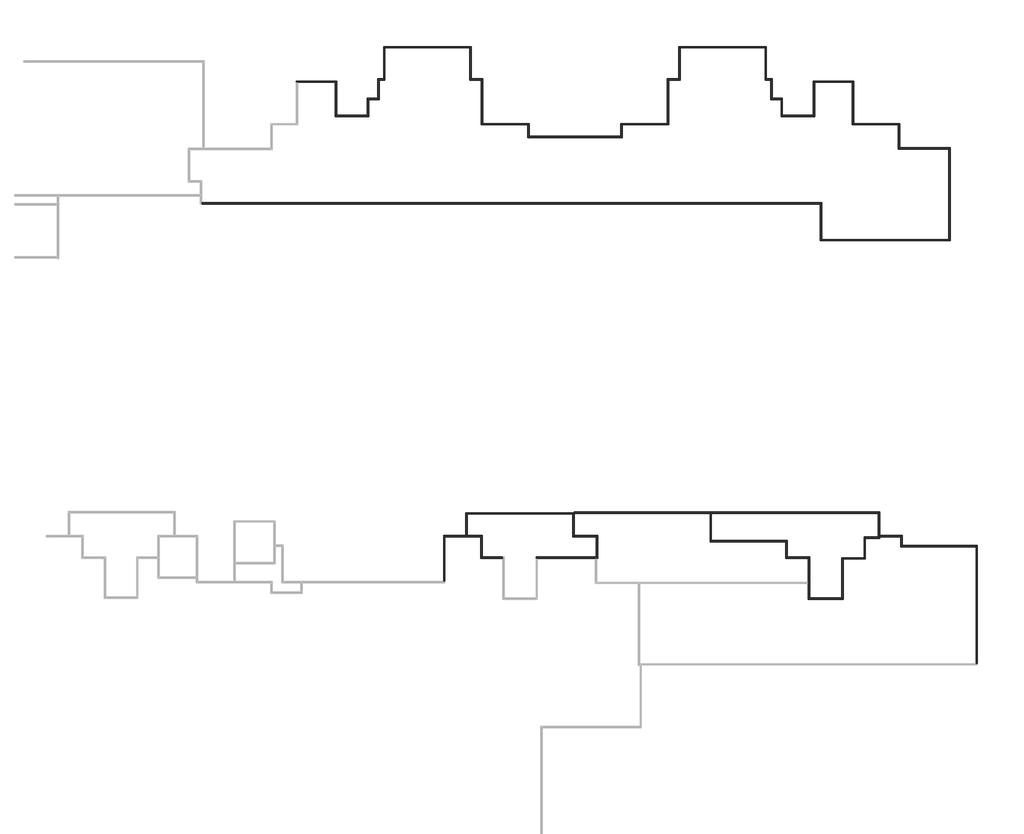
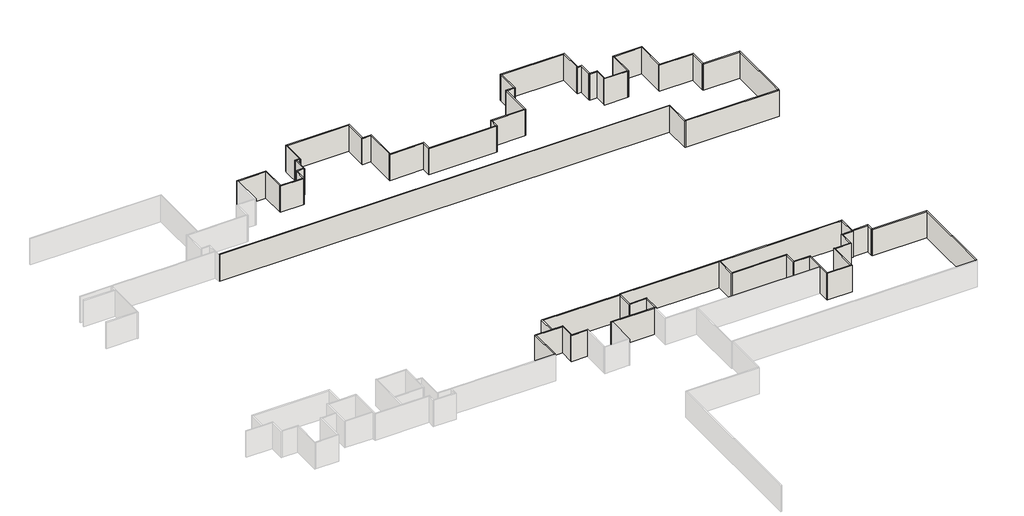
# One storey, part 8 of 8: 63 walls.
"""IFC4 building model written with IfcOpenShell, lengths in millimetres."""

import ifcopenshell
import ifcopenshell.guid

model = None  # the IFC model being written
_history = None  # IfcOwnerHistory: only IFC2X3 demands one
_inside = {}  # id of a spatial element -> (the spatial element, [elements in it])
_under = {}  # id of a project, library or spatial element -> (it, [spatial elements below it])
_declared = {}  # id of a project -> (the project, [libraries it declares])
_typed = {}  # id of a type object -> (the type object, [elements of that type])
_made_of = {}  # id of a material, layer set ... -> (it, [elements and type objects made of it])


def new_model(schema):
    """Start an empty IFC model of exactly this schema.

    Asked for "IFC4X3", IfcOpenShell would pick the latest addendum, in which some entities
    have other attributes; the version numbers below select the first issue.
    IFC2X3 requires an IfcOwnerHistory on every rooted entity: one is made here for all.
    """
    global model, _history
    if schema == "IFC4X3":
        model = ifcopenshell.file(schema_version=(4, 3, 0, 0))
    else:
        model = ifcopenshell.file(schema=schema)
    _inside.clear()
    _under.clear()
    _declared.clear()
    _typed.clear()
    _made_of.clear()
    _history = None
    if model.schema == "IFC2X3":
        org = make("IfcOrganization", Name="unknown")
        user = make(
            "IfcPersonAndOrganization",
            ThePerson=make("IfcPerson", FamilyName="unknown"),
            TheOrganization=org,
        )
        app = make(
            "IfcApplication",
            ApplicationDeveloper=org,
            Version="unknown",
            ApplicationFullName="unknown",
            ApplicationIdentifier="unknown",
        )
        _history = make(
            "IfcOwnerHistory",
            OwningUser=user,
            OwningApplication=app,
            ChangeAction="ADDED",
            CreationDate=0,
        )
    return model


def make(cls, **values):
    """One entity of the class cls with the attributes given. An attribute that is None is left unset."""
    return model.create_entity(
        cls, **{name: value for name, value in values.items() if value is not None}
    )


def rooted(cls, **values):
    """An entity with a GlobalId (a new one), such as an element, a storey or a relation."""
    return make(cls, GlobalId=ifcopenshell.guid.new(), OwnerHistory=_history, **values)


def si_unit(unit_type, name, prefix=None):
    """IfcSIUnit, for example si_unit("LENGTHUNIT", "METRE", prefix="MILLI")."""
    return make("IfcSIUnit", UnitType=unit_type, Prefix=prefix, Name=name)


def assignment(units):
    """IfcUnitAssignment: the units of a project."""
    return None if units is None else make("IfcUnitAssignment", Units=units)


def point(xyz):
    """IfcCartesianPoint."""
    return None if xyz is None else make("IfcCartesianPoint", Coordinates=xyz)


def direction(xyz):
    """IfcDirection."""
    return None if xyz is None else make("IfcDirection", DirectionRatios=xyz)


def frame(location, z_axis=None, x_axis=None):
    """IfcAxis2Placement3D, a coordinate frame: its origin and axes. An axis left out is left unset."""
    return make(
        "IfcAxis2Placement3D",
        Location=point(location),
        Axis=direction(z_axis),
        RefDirection=direction(x_axis),
    )


def origin():
    """The frame at (0, 0, 0) with its axes left unset."""
    return frame((0.0, 0.0, 0.0))


def origin_with_axes():
    """The frame at (0, 0, 0) with the z axis (0, 0, 1) and the x axis (1, 0, 0) written out."""
    return frame((0.0, 0.0, 0.0), z_axis=(0.0, 0.0, 1.0), x_axis=(1.0, 0.0, 0.0))


def place(relative_to, where):
    """IfcLocalPlacement: puts the frame where relative to a parent placement (None: the world)."""
    return make(
        "IfcLocalPlacement", PlacementRelTo=relative_to, RelativePlacement=where
    )


def context(
    kind, dimensions, precision=None, world=None, true_north=None, identifier=None
):
    """IfcGeometricRepresentationContext, for example the 3D "Model" context."""
    return make(
        "IfcGeometricRepresentationContext",
        ContextIdentifier=identifier,
        ContextType=kind,
        CoordinateSpaceDimension=dimensions,
        Precision=precision,
        WorldCoordinateSystem=world,
        TrueNorth=true_north,
    )


def project(units=None, contexts=None):
    """IfcProject with its units and contexts."""
    return rooted(
        "IfcProject",
        Name="project",
        RepresentationContexts=contexts,
        UnitsInContext=assignment(units),
    )


def spatial(cls, under=None, at=None, **own):
    """A site, building, storey or space (cls), placed at a placement, below another one or the project."""
    s = rooted(cls, ObjectPlacement=at, **own)
    if under is not None:
        _under.setdefault(under.id(), (under, []))[1].append(s)
    return s


def polyline(points):
    """IfcPolyline through the points."""
    return make("IfcPolyline", Points=[point(p) for p in points])


def outline(outer, holes=None, kind="AREA"):
    """IfcArbitraryClosedProfileDef: a profile drawn as a closed curve; with holes, ...WithVoids."""
    if holes is None:
        return make("IfcArbitraryClosedProfileDef", ProfileType=kind, OuterCurve=outer)
    return make(
        "IfcArbitraryProfileDefWithVoids",
        ProfileType=kind,
        OuterCurve=outer,
        InnerCurves=holes,
    )


def extrude(swept, where, along, depth):
    """IfcExtrudedAreaSolid: the profile swept, set in the frame where, extruded along a direction by depth."""
    return make(
        "IfcExtrudedAreaSolid",
        SweptArea=swept,
        Position=where,
        ExtrudedDirection=direction(along),
        Depth=depth,
    )


def faces_of(points, faces, orient=None, outer=None):
    """IfcFace entities. A face is a list of loops; a loop is a list of indices into points, from 0.

    orient and outer hold one flag for each loop. By default every Orientation is true, the
    first loop of a face is its IfcFaceOuterBound and the others are IfcFaceBound.
    """
    made = []
    for i, loops in enumerate(faces):
        bounds = []
        for j, loop in enumerate(loops):
            is_outer = j == 0 if outer is None else outer[i][j]
            bounds.append(
                make(
                    "IfcFaceOuterBound" if is_outer else "IfcFaceBound",
                    Bound=make("IfcPolyLoop", Polygon=[points[k] for k in loop]),
                    Orientation=True if orient is None else orient[i][j],
                )
            )
        made.append(make("IfcFace", Bounds=bounds))
    return made


def faceted_brep(points, faces, orient=None, outer=None, voids=None):
    """IfcFacetedBrep: a solid bounded by flat faces; with voids (closed shells), ...WithVoids."""
    shared = [point(p) for p in points]
    hull = make("IfcClosedShell", CfsFaces=faces_of(shared, faces, orient, outer))
    if voids is None:
        return make("IfcFacetedBrep", Outer=hull)
    return make(
        "IfcFacetedBrepWithVoids",
        Outer=hull,
        Voids=[
            make(cls, CfsFaces=faces_of(shared, fs, o, b)) for cls, fs, o, b in voids
        ],
    )


def shape(context_of_items, identifier, shape_type, items):
    """IfcShapeRepresentation: the items that make up one representation, for example the "Body"."""
    return make(
        "IfcShapeRepresentation",
        ContextOfItems=context_of_items,
        RepresentationIdentifier=identifier,
        RepresentationType=shape_type,
        Items=items,
    )


def made_of(thing, what):
    """Note that an element or type object is made of a material, layer set ...; save() writes the relation."""
    if what is not None:
        _made_of.setdefault(what.id(), (what, []))[1].append(thing)
    return thing


def element(
    cls,
    number,
    at=None,
    inside=None,
    cuts=None,
    type_object=None,
    material=None,
    context=None,
    identifier="Body",
    shape_type=None,
    held_by="IfcProductDefinitionShape",
    body=None,
    shapes=None,
    **own,
):
    """One element of the class cls, such as IfcWall. Its Tag is "e" and its number.

    at: its placement. inside: the storey or other place that contains it. cuts: it is an
    opening in that element (IfcRelVoidsElement). A single representation is given by context,
    identifier, shape_type and body (its items); several are given by shapes. held_by: the class
    of the entity that holds the representations. save() writes the other relations.
    """
    e = rooted(cls, Tag="e%d" % number, ObjectPlacement=at, **own)
    if body is not None:
        shapes = [shape(context, identifier, shape_type, body)]
    if shapes is not None:
        e.Representation = make(held_by, Representations=shapes)
    if inside is not None:
        _inside.setdefault(inside.id(), (inside, []))[1].append(e)
    if cuts is not None:
        rooted(
            "IfcRelVoidsElement", RelatingBuildingElement=cuts, RelatedOpeningElement=e
        )
    if type_object is not None:
        _typed.setdefault(type_object.id(), (type_object, []))[1].append(e)
    return made_of(e, material)


def aggregate(whole, parts):
    """IfcRelAggregates: a whole, such as a stair, and the parts it consists of."""
    return rooted("IfcRelAggregates", RelatingObject=whole, RelatedObjects=parts)


def save(model, path):
    """Write the relations noted so far, then the file.

    IfcRelAggregates (storeys below a building ...), IfcRelContainedInSpatialStructure (elements
    in a storey), IfcRelDefinesByType, IfcRelAssociatesMaterial and IfcRelDeclares: one each for
    every whole, place, type object, material and project.
    """
    for whole, parts in _under.values():
        aggregate(whole, parts)
    for where, things in _inside.values():
        rooted(
            "IfcRelContainedInSpatialStructure",
            RelatedElements=things,
            RelatingStructure=where,
        )
    for kind, things in _typed.values():
        rooted("IfcRelDefinesByType", RelatedObjects=things, RelatingType=kind)
    for what, things in _made_of.values():
        rooted("IfcRelAssociatesMaterial", RelatedObjects=things, RelatingMaterial=what)
    for by, libraries in _declared.values():
        rooted("IfcRelDeclares", RelatingContext=by, RelatedDefinitions=libraries)
    model.write(path)


model = new_model("IFC4")

# Units and contexts
model_context = context("Model", 3, world=origin())
ifc_project = project(units=[si_unit("LENGTHUNIT", "METRE", prefix="MILLI")], contexts=[model_context])

# Site, building, storey
site = spatial("IfcSite", under=ifc_project)
building = spatial("IfcBuilding", under=site)
storey = spatial("IfcBuildingStorey", under=building, Name="户型图", Elevation=0.0)

# Walls
placement = place(None, origin())
element("IfcWall", 1, ObjectType="所有墙体", at=placement, inside=storey, context=model_context, shape_type="Brep", body=[
    faceted_brep([(247659.8041272, 127629.6486698, 0.0), (301497.9590704, 127629.6486698, 0.0), (301617.9590704, 127629.6486698, 0.0), (301617.9590704, 127629.6486698, 3300.0), (301497.9590704, 127629.6486698, 3300.0), (247659.8041272, 127629.6486698, 3300.0), (247659.8041272, 127749.6486698, 0.0), (247659.8041272, 127749.6486698, 3300.0), (301617.9590704, 127749.6486698, 3300.0), (301617.9590704, 127749.6486698, 0.0)], [[[0, 1, 2, 3, 4, 5]], [[6, 7, 8, 9]], [[2, 1, 0, 6, 9]], [[5, 4, 3, 8, 7]], [[0, 5, 7, 6]], [[3, 2, 9, 8]]]),
])
element("IfcWall", 2, ObjectType="所有墙体", at=placement, inside=storey, context=model_context, shape_type="Brep", body=[
    faceted_brep([(301497.9590704, 127629.6486698, 0.0), (301497.9590704, 124429.6486698, 0.0), (301497.9590704, 124429.6486698, 3300.0), (301497.9590704, 127629.6486698, 3300.0), (301617.9590704, 127629.6486698, 0.0), (301617.9590704, 127629.6486698, 3300.0), (301617.9590704, 124549.6486698, 3300.0), (301617.9590704, 124429.6486698, 3300.0), (301617.9590704, 124429.6486698, 0.0), (301617.9590704, 124549.6486698, 0.0)], [[[0, 1, 2, 3]], [[4, 5, 6, 7, 8, 9]], [[1, 0, 4, 9, 8]], [[3, 2, 7, 6, 5]], [[0, 3, 5, 4]], [[2, 1, 8, 7]]]),
])
element("IfcWall", 3, ObjectType="所有墙体", at=placement, inside=storey, context=model_context, shape_type="Brep", body=[
    faceted_brep([(301617.9590704, 124429.6486698, 0.0), (312809.8041272, 124429.6486698, 0.0), (312809.8041272, 124429.6486698, 3300.0), (301617.9590704, 124429.6486698, 3300.0), (301617.9590704, 124549.6486698, 0.0), (301617.9590704, 124549.6486698, 3300.0), (312689.8041272, 124549.6486698, 3300.0), (312809.8041272, 124549.6486698, 3300.0), (312809.8041272, 124549.6486698, 0.0), (312689.8041272, 124549.6486698, 0.0)], [[[0, 1, 2, 3]], [[4, 5, 6, 7, 8, 9]], [[1, 0, 4, 9, 8]], [[3, 2, 7, 6, 5]], [[0, 3, 5, 4]], [[2, 1, 8, 7]]]),
])
element("IfcWall", 4, ObjectType="所有墙体", at=placement, inside=storey, context=model_context, shape_type="Brep", body=[
    faceted_brep([(312809.8041272, 124549.6486698, 0.0), (312809.8041272, 132549.6486698, 0.0), (312809.8041272, 132549.6486698, 3300.0), (312809.8041272, 124549.6486698, 3300.0), (312689.8041272, 124549.6486698, 0.0), (312689.8041272, 124549.6486698, 3300.0), (312689.8041272, 132429.6486698, 3300.0), (312689.8041272, 132549.6486698, 3300.0), (312689.8041272, 132549.6486698, 0.0), (312689.8041272, 132429.6486698, 0.0)], [[[0, 1, 2, 3]], [[4, 5, 6, 7, 8, 9]], [[1, 0, 4, 9, 8]], [[3, 2, 7, 6, 5]], [[0, 3, 5, 4]], [[2, 1, 8, 7]]]),
])
element("IfcWall", 5, ObjectType="所有墙体", at=placement, inside=storey, context=model_context, shape_type="Brep", body=[
    faceted_brep([(312689.8041272, 132549.6486698, 0.0), (308409.8041268, 132549.6486698, 0.0), (308289.8041268, 132549.6486698, 0.0), (308289.8041268, 132549.6486698, 3300.0), (308409.8041268, 132549.6486698, 3300.0), (312689.8041272, 132549.6486698, 3300.0), (312689.8041272, 132429.6486698, 0.0), (312689.8041272, 132429.6486698, 3300.0), (308289.8041268, 132429.6486698, 3300.0), (308289.8041268, 132429.6486698, 0.0)], [[[0, 1, 2, 3, 4, 5]], [[6, 7, 8, 9]], [[2, 1, 0, 6, 9]], [[5, 4, 3, 8, 7]], [[0, 5, 7, 6]], [[3, 2, 9, 8]]]),
])
element("IfcWall", 6, ObjectType="所有墙体", at=placement, inside=storey, context=model_context, shape_type="Brep", body=[
    faceted_brep([(308409.8041268, 132549.6486698, 0.0), (308409.8041268, 134649.648667, 0.0), (308409.8041268, 134649.648667, 3300.0), (308409.8041268, 132549.6486698, 3300.0), (308289.8041268, 132549.6486698, 0.0), (308289.8041268, 132549.6486698, 3300.0), (308289.8041268, 134529.648667, 3300.0), (308289.8041268, 134649.648667, 3300.0), (308289.8041268, 134649.648667, 0.0), (308289.8041268, 134529.648667, 0.0)], [[[0, 1, 2, 3]], [[4, 5, 6, 7, 8, 9]], [[1, 0, 4, 9, 8]], [[3, 2, 7, 6, 5]], [[0, 3, 5, 4]], [[2, 1, 8, 7]]]),
])
element("IfcWall", 7, ObjectType="所有墙体", at=placement, inside=storey, context=model_context, shape_type="Brep", body=[
    faceted_brep([(308289.8041268, 134649.648667, 0.0), (304409.8041273, 134649.648667, 0.0), (304289.8041273, 134649.648667, 0.0), (304289.8041273, 134649.648667, 3300.0), (304409.8041273, 134649.648667, 3300.0), (308289.8041268, 134649.648667, 3300.0), (308289.8041268, 134529.648667, 0.0), (308289.8041268, 134529.648667, 3300.0), (304289.8041273, 134529.648667, 3300.0), (304289.8041273, 134529.648667, 0.0)], [[[0, 1, 2, 3, 4, 5]], [[6, 7, 8, 9]], [[2, 1, 0, 6, 9]], [[5, 4, 3, 8, 7]], [[0, 5, 7, 6]], [[3, 2, 9, 8]]]),
])
element("IfcWall", 8, ObjectType="所有墙体", at=placement, inside=storey, context=model_context, shape_type="Brep", body=[
    faceted_brep([(304409.8041273, 134649.648667, 0.0), (304409.8041273, 138349.6486699, 0.0), (304409.8041273, 138349.6486699, 3300.0), (304409.8041273, 134649.648667, 3300.0), (304289.8041273, 134649.648667, 0.0), (304289.8041273, 134649.648667, 3300.0), (304289.8041273, 138229.6486699, 3300.0), (304289.8041273, 138349.6486699, 3300.0), (304289.8041273, 138349.6486699, 0.0), (304289.8041273, 138229.6486699, 0.0)], [[[0, 1, 2, 3]], [[4, 5, 6, 7, 8, 9]], [[1, 0, 4, 9, 8]], [[3, 2, 7, 6, 5]], [[0, 3, 5, 4]], [[2, 1, 8, 7]]]),
])
element("IfcWall", 9, ObjectType="所有墙体", at=placement, inside=storey, context=model_context, shape_type="Brep", body=[
    faceted_brep([(304289.8041273, 138349.6486699, 0.0), (300889.8041266, 138349.6486699, 0.0), (300889.8041266, 138349.6486699, 3300.0), (304289.8041273, 138349.6486699, 3300.0), (304289.8041273, 138229.6486699, 0.0), (304289.8041273, 138229.6486699, 3300.0), (301009.8041266, 138229.6486699, 3300.0), (300889.8041266, 138229.6486699, 3300.0), (300889.8041266, 138229.6486699, 0.0), (301009.8041266, 138229.6486699, 0.0)], [[[0, 1, 2, 3]], [[4, 5, 6, 7, 8, 9]], [[1, 0, 4, 9, 8]], [[3, 2, 7, 6, 5]], [[0, 3, 5, 4]], [[2, 1, 8, 7]]]),
])
element("IfcWall", 10, ObjectType="所有墙体", at=placement, inside=storey, context=model_context, shape_type="Brep", body=[
    faceted_brep([(300889.8041266, 138229.6486699, 0.0), (300889.8041266, 135349.6486699, 0.0), (300889.8041266, 135229.6486699, 0.0), (300889.8041266, 135229.6486699, 3300.0), (300889.8041266, 135349.6486699, 3300.0), (300889.8041266, 138229.6486699, 3300.0), (301009.8041266, 138229.6486699, 0.0), (301009.8041266, 138229.6486699, 3300.0), (301009.8041266, 135229.6486699, 3300.0), (301009.8041266, 135229.6486699, 0.0)], [[[0, 1, 2, 3, 4, 5]], [[6, 7, 8, 9]], [[2, 1, 0, 6, 9]], [[5, 4, 3, 8, 7]], [[0, 5, 7, 6]], [[3, 2, 9, 8]]]),
])
element("IfcWall", 11, ObjectType="所有墙体", at=placement, inside=storey, context=model_context, shape_type="Brep", body=[
    faceted_brep([(300889.8041266, 135349.6486699, 0.0), (298209.5033683, 135349.6486699, 0.0), (298089.5033683, 135349.6486699, 0.0), (298089.5033683, 135349.6486699, 3300.0), (298209.5033683, 135349.6486699, 3300.0), (300889.8041266, 135349.6486699, 3300.0), (300889.8041266, 135229.6486699, 0.0), (300889.8041266, 135229.6486699, 3300.0), (298089.5033683, 135229.6486699, 3300.0), (298089.5033683, 135229.6486699, 0.0)], [[[0, 1, 2, 3, 4, 5]], [[6, 7, 8, 9]], [[2, 1, 0, 6, 9]], [[5, 4, 3, 8, 7]], [[0, 5, 7, 6]], [[3, 2, 9, 8]]]),
])
element("IfcWall", 12, ObjectType="所有墙体", at=placement, inside=storey, context=model_context, shape_type="Brep", body=[
    faceted_brep([(298209.5033683, 135349.6486699, 0.0), (298209.5033683, 136849.6486657, 0.0), (298209.5033683, 136849.6486657, 3300.0), (298209.5033683, 135349.6486699, 3300.0), (298089.5033683, 135349.6486699, 0.0), (298089.5033683, 135349.6486699, 3300.0), (298089.5033683, 136729.6486657, 3300.0), (298089.5033683, 136849.6486657, 3300.0), (298089.5033683, 136849.6486657, 0.0), (298089.5033683, 136729.6486657, 0.0)], [[[0, 1, 2, 3]], [[4, 5, 6, 7, 8, 9]], [[1, 0, 4, 9, 8]], [[3, 2, 7, 6, 5]], [[0, 3, 5, 4]], [[2, 1, 8, 7]]]),
])
element("IfcWall", 13, ObjectType="所有墙体", at=placement, inside=storey, context=model_context, shape_type="Brep", body=[
    faceted_brep([(298089.5033683, 136849.6486657, 0.0), (297309.8041265, 136849.6486657, 0.0), (297189.8041265, 136849.6486657, 0.0), (297189.8041265, 136849.6486657, 3300.0), (297309.8041265, 136849.6486657, 3300.0), (298089.5033683, 136849.6486657, 3300.0), (298089.5033683, 136729.6486657, 0.0), (298089.5033683, 136729.6486657, 3300.0), (297189.8041265, 136729.6486657, 3300.0), (297189.8041265, 136729.6486657, 0.0)], [[[0, 1, 2, 3, 4, 5]], [[6, 7, 8, 9]], [[2, 1, 0, 6, 9]], [[5, 4, 3, 8, 7]], [[0, 5, 7, 6]], [[3, 2, 9, 8]]]),
])
element("IfcWall", 14, ObjectType="所有墙体", at=placement, inside=storey, context=model_context, shape_type="Brep", body=[
    faceted_brep([(297309.8041265, 136849.6486657, 0.0), (297309.8041265, 138549.6486701, 0.0), (297309.8041265, 138549.6486701, 3300.0), (297309.8041265, 136849.6486657, 3300.0), (297189.8041265, 136849.6486657, 0.0), (297189.8041265, 136849.6486657, 3300.0), (297189.8041265, 138429.6486701, 3300.0), (297189.8041265, 138549.6486701, 3300.0), (297189.8041265, 138549.6486701, 0.0), (297189.8041265, 138429.6486701, 0.0)], [[[0, 1, 2, 3]], [[4, 5, 6, 7, 8, 9]], [[1, 0, 4, 9, 8]], [[3, 2, 7, 6, 5]], [[0, 3, 5, 4]], [[2, 1, 8, 7]]]),
])
element("IfcWall", 15, ObjectType="所有墙体", at=placement, inside=storey, context=model_context, shape_type="Brep", body=[
    faceted_brep([(297189.8041265, 138549.6486701, 0.0), (296809.8041265, 138549.6486701, 0.0), (296689.8041265, 138549.6486701, 0.0), (296689.8041265, 138549.6486701, 3300.0), (296809.8041265, 138549.6486701, 3300.0), (297189.8041265, 138549.6486701, 3300.0), (297189.8041265, 138429.6486701, 0.0), (297189.8041265, 138429.6486701, 3300.0), (296689.8041265, 138429.6486701, 3300.0), (296689.8041265, 138429.6486701, 0.0)], [[[0, 1, 2, 3, 4, 5]], [[6, 7, 8, 9]], [[2, 1, 0, 6, 9]], [[5, 4, 3, 8, 7]], [[0, 5, 7, 6]], [[3, 2, 9, 8]]]),
])
element("IfcWall", 16, ObjectType="所有墙体", at=placement, inside=storey, context=model_context, shape_type="Brep", body=[
    faceted_brep([(296809.8041265, 138549.6486701, 0.0), (296809.8041265, 141349.6486699, 0.0), (296809.8041265, 141349.6486699, 3300.0), (296809.8041265, 138549.6486701, 3300.0), (296689.8041265, 138549.6486701, 0.0), (296689.8041265, 138549.6486701, 3300.0), (296689.8041265, 141229.6486699, 3300.0), (296689.8041265, 141349.6486699, 3300.0), (296689.8041265, 141349.6486699, 0.0), (296689.8041265, 141229.6486699, 0.0)], [[[0, 1, 2, 3]], [[4, 5, 6, 7, 8, 9]], [[1, 0, 4, 9, 8]], [[3, 2, 7, 6, 5]], [[0, 3, 5, 4]], [[2, 1, 8, 7]]]),
])
element("IfcWall", 17, ObjectType="所有墙体", at=placement, inside=storey, context=model_context, shape_type="Brep", body=[
    faceted_brep([(296689.8041265, 141349.6486699, 0.0), (289189.8041265, 141349.6486699, 0.0), (289189.8041265, 141349.6486699, 3300.0), (296689.8041265, 141349.6486699, 3300.0), (296689.8041265, 141229.6486699, 0.0), (296689.8041265, 141229.6486699, 3300.0), (289309.8041265, 141229.6486699, 3300.0), (289189.8041265, 141229.6486699, 3300.0), (289189.8041265, 141229.6486699, 0.0), (289309.8041265, 141229.6486699, 0.0)], [[[0, 1, 2, 3]], [[4, 5, 6, 7, 8, 9]], [[1, 0, 4, 9, 8]], [[3, 2, 7, 6, 5]], [[0, 3, 5, 4]], [[2, 1, 8, 7]]]),
])
element("IfcWall", 18, ObjectType="所有墙体", at=placement, inside=storey, context=model_context, shape_type="Brep", body=[
    faceted_brep([(289189.8041265, 141229.6486699, 0.0), (289189.8041265, 138549.6486701, 0.0), (289189.8041265, 138429.6486701, 0.0), (289189.8041265, 138429.6486701, 3300.0), (289189.8041265, 138549.6486701, 3300.0), (289189.8041265, 141229.6486699, 3300.0), (289309.8041265, 141229.6486699, 0.0), (289309.8041265, 141229.6486699, 3300.0), (289309.8041265, 138429.6486701, 3300.0), (289309.8041265, 138429.6486701, 0.0)], [[[0, 1, 2, 3, 4, 5]], [[6, 7, 8, 9]], [[2, 1, 0, 6, 9]], [[5, 4, 3, 8, 7]], [[0, 5, 7, 6]], [[3, 2, 9, 8]]]),
])
element("IfcWall", 19, ObjectType="所有墙体", at=placement, inside=storey, context=model_context, shape_type="Brep", body=[
    faceted_brep([(289189.8041265, 138549.6486701, 0.0), (288186.9696276, 138549.6486701, 0.0), (288186.9696276, 138549.6486701, 3300.0), (289189.8041265, 138549.6486701, 3300.0), (289189.8041265, 138429.6486701, 0.0), (289189.8041265, 138429.6486701, 3300.0), (288306.9696276, 138429.6486701, 3300.0), (288186.9696276, 138429.6486701, 3300.0), (288186.9696276, 138429.6486701, 0.0), (288306.9696276, 138429.6486701, 0.0)], [[[0, 1, 2, 3]], [[4, 5, 6, 7, 8, 9]], [[1, 0, 4, 9, 8]], [[3, 2, 7, 6, 5]], [[0, 3, 5, 4]], [[2, 1, 8, 7]]]),
])
element("IfcWall", 20, ObjectType="所有墙体", at=placement, inside=storey, context=model_context, shape_type="Brep", body=[
    faceted_brep([(288186.9696276, 138429.6486701, 0.0), (288186.9696276, 134649.648667, 0.0), (288186.9696276, 134529.648667, 0.0), (288186.9696276, 134529.648667, 3300.0), (288186.9696276, 134649.648667, 3300.0), (288186.9696276, 138429.6486701, 3300.0), (288306.9696276, 138429.6486701, 0.0), (288306.9696276, 138429.6486701, 3300.0), (288306.9696276, 134529.648667, 3300.0), (288306.9696276, 134529.648667, 0.0)], [[[0, 1, 2, 3, 4, 5]], [[6, 7, 8, 9]], [[2, 1, 0, 6, 9]], [[5, 4, 3, 8, 7]], [[0, 5, 7, 6]], [[3, 2, 9, 8]]]),
])
element("IfcWall", 21, ObjectType="所有墙体", at=placement, inside=storey, context=model_context, shape_type="Brep", body=[
    faceted_brep([(288186.9696276, 134649.648667, 0.0), (284139.8041273, 134649.648667, 0.0), (284139.8041273, 134649.648667, 3300.0), (288186.9696276, 134649.648667, 3300.0), (288186.9696276, 134529.648667, 0.0), (288186.9696276, 134529.648667, 3300.0), (284259.8041273, 134529.648667, 3300.0), (284139.8041273, 134529.648667, 3300.0), (284139.8041273, 134529.648667, 0.0), (284259.8041273, 134529.648667, 0.0)], [[[0, 1, 2, 3]], [[4, 5, 6, 7, 8, 9]], [[1, 0, 4, 9, 8]], [[3, 2, 7, 6, 5]], [[0, 3, 5, 4]], [[2, 1, 8, 7]]]),
])
element("IfcWall", 22, ObjectType="所有墙体", at=placement, inside=storey, context=model_context, shape_type="Brep", body=[
    faceted_brep([(284139.8041273, 134529.648667, 0.0), (284139.8041273, 133549.6486685, 0.0), (284139.8041273, 133429.6486685, 0.0), (284139.8041273, 133429.6486685, 3300.0), (284139.8041273, 133549.6486685, 3300.0), (284139.8041273, 134529.648667, 3300.0), (284259.8041273, 134529.648667, 0.0), (284259.8041273, 134529.648667, 3300.0), (284259.8041273, 133429.6486685, 3300.0), (284259.8041273, 133429.6486685, 0.0)], [[[0, 1, 2, 3, 4, 5]], [[6, 7, 8, 9]], [[2, 1, 0, 6, 9]], [[5, 4, 3, 8, 7]], [[0, 5, 7, 6]], [[3, 2, 9, 8]]]),
])
element("IfcWall", 23, ObjectType="所有墙体", at=placement, inside=storey, context=model_context, shape_type="Brep", body=[
    faceted_brep([(284139.8041273, 133549.6486685, 0.0), (276159.8041272, 133549.6486685, 0.0), (276039.8041272, 133549.6486685, 0.0), (276039.8041272, 133549.6486685, 3300.0), (276159.8041272, 133549.6486685, 3300.0), (284139.8041273, 133549.6486685, 3300.0), (284139.8041273, 133429.6486685, 0.0), (284139.8041273, 133429.6486685, 3300.0), (276039.8041272, 133429.6486685, 3300.0), (276039.8041272, 133429.6486685, 0.0)], [[[0, 1, 2, 3, 4, 5]], [[6, 7, 8, 9]], [[2, 1, 0, 6, 9]], [[5, 4, 3, 8, 7]], [[0, 5, 7, 6]], [[3, 2, 9, 8]]]),
])
element("IfcWall", 24, ObjectType="所有墙体", at=placement, inside=storey, context=model_context, shape_type="Brep", body=[
    faceted_brep([(276159.8041272, 133549.6486685, 0.0), (276159.8041272, 134649.648667, 0.0), (276159.8041272, 134649.648667, 3300.0), (276159.8041272, 133549.6486685, 3300.0), (276039.8041272, 133549.6486685, 0.0), (276039.8041272, 133549.6486685, 3300.0), (276039.8041272, 134529.648667, 3300.0), (276039.8041272, 134649.648667, 3300.0), (276039.8041272, 134649.648667, 0.0), (276039.8041272, 134529.648667, 0.0)], [[[0, 1, 2, 3]], [[4, 5, 6, 7, 8, 9]], [[1, 0, 4, 9, 8]], [[3, 2, 7, 6, 5]], [[0, 3, 5, 4]], [[2, 1, 8, 7]]]),
])
element("IfcWall", 25, ObjectType="所有墙体", at=placement, inside=storey, context=model_context, shape_type="Brep", body=[
    faceted_brep([(276039.8041272, 134649.648667, 0.0), (272109.8715566, 134649.648667, 0.0), (271989.8715566, 134649.648667, 0.0), (271989.8715566, 134649.648667, 3300.0), (272109.8715566, 134649.648667, 3300.0), (276039.8041272, 134649.648667, 3300.0), (276039.8041272, 134529.648667, 0.0), (276039.8041272, 134529.648667, 3300.0), (271989.8715566, 134529.648667, 3300.0), (271989.8715566, 134529.648667, 0.0)], [[[0, 1, 2, 3, 4, 5]], [[6, 7, 8, 9]], [[2, 1, 0, 6, 9]], [[5, 4, 3, 8, 7]], [[0, 5, 7, 6]], [[3, 2, 9, 8]]]),
])
element("IfcWall", 26, ObjectType="所有墙体", at=placement, inside=storey, context=model_context, shape_type="Brep", body=[
    faceted_brep([(272109.8715566, 134649.648667, 0.0), (272109.8715566, 138549.6486701, 0.0), (272109.8715566, 138549.6486701, 3300.0), (272109.8715566, 134649.648667, 3300.0), (271989.8715566, 134649.648667, 0.0), (271989.8715566, 134649.648667, 3300.0), (271989.8715566, 138429.6486701, 3300.0), (271989.8715566, 138549.6486701, 3300.0), (271989.8715566, 138549.6486701, 0.0), (271989.8715566, 138429.6486701, 0.0)], [[[0, 1, 2, 3]], [[4, 5, 6, 7, 8, 9]], [[1, 0, 4, 9, 8]], [[3, 2, 7, 6, 5]], [[0, 3, 5, 4]], [[2, 1, 8, 7]]]),
])
element("IfcWall", 27, ObjectType="所有墙体", at=placement, inside=storey, context=model_context, shape_type="Brep", body=[
    faceted_brep([(271989.8715566, 138549.6486701, 0.0), (271109.8041271, 138549.6486701, 0.0), (270989.8041271, 138549.6486701, 0.0), (270989.8041271, 138549.6486701, 3300.0), (271109.8041271, 138549.6486701, 3300.0), (271989.8715566, 138549.6486701, 3300.0), (271989.8715566, 138429.6486701, 0.0), (271989.8715566, 138429.6486701, 3300.0), (270989.8041271, 138429.6486701, 3300.0), (270989.8041271, 138429.6486701, 0.0)], [[[0, 1, 2, 3, 4, 5]], [[6, 7, 8, 9]], [[2, 1, 0, 6, 9]], [[5, 4, 3, 8, 7]], [[0, 5, 7, 6]], [[3, 2, 9, 8]]]),
])
element("IfcWall", 28, ObjectType="所有墙体", at=placement, inside=storey, context=model_context, shape_type="Brep", body=[
    faceted_brep([(271109.8041271, 138549.6486701, 0.0), (271109.8041271, 141349.6486699, 0.0), (271109.8041271, 141349.6486699, 3300.0), (271109.8041271, 138549.6486701, 3300.0), (270989.8041271, 138549.6486701, 0.0), (270989.8041271, 138549.6486701, 3300.0), (270989.8041271, 141229.6486699, 3300.0), (270989.8041271, 141349.6486699, 3300.0), (270989.8041271, 141349.6486699, 0.0), (270989.8041271, 141229.6486699, 0.0)], [[[0, 1, 2, 3]], [[4, 5, 6, 7, 8, 9]], [[1, 0, 4, 9, 8]], [[3, 2, 7, 6, 5]], [[0, 3, 5, 4]], [[2, 1, 8, 7]]]),
])
element("IfcWall", 29, ObjectType="所有墙体", at=placement, inside=storey, context=model_context, shape_type="Brep", body=[
    faceted_brep([(270989.8041271, 141349.6486699, 0.0), (263489.8041272, 141349.6486699, 0.0), (263489.8041272, 141349.6486699, 3300.0), (270989.8041271, 141349.6486699, 3300.0), (270989.8041271, 141229.6486699, 0.0), (270989.8041271, 141229.6486699, 3300.0), (263609.8041272, 141229.6486699, 3300.0), (263489.8041272, 141229.6486699, 3300.0), (263489.8041272, 141229.6486699, 0.0), (263609.8041272, 141229.6486699, 0.0)], [[[0, 1, 2, 3]], [[4, 5, 6, 7, 8, 9]], [[1, 0, 4, 9, 8]], [[3, 2, 7, 6, 5]], [[0, 3, 5, 4]], [[2, 1, 8, 7]]]),
])
element("IfcWall", 30, ObjectType="所有墙体", at=placement, inside=storey, context=model_context, shape_type="Brep", body=[
    faceted_brep([(263489.8041272, 141229.6486699, 0.0), (263489.8041272, 138549.6486701, 0.0), (263489.8041272, 138429.6486701, 0.0), (263489.8041272, 138429.6486701, 3300.0), (263489.8041272, 138549.6486701, 3300.0), (263489.8041272, 141229.6486699, 3300.0), (263609.8041272, 141229.6486699, 0.0), (263609.8041272, 141229.6486699, 3300.0), (263609.8041272, 138429.6486701, 3300.0), (263609.8041272, 138429.6486701, 0.0)], [[[0, 1, 2, 3, 4, 5]], [[6, 7, 8, 9]], [[2, 1, 0, 6, 9]], [[5, 4, 3, 8, 7]], [[0, 5, 7, 6]], [[3, 2, 9, 8]]]),
])
element("IfcWall", 31, ObjectType="所有墙体", at=placement, inside=storey, context=model_context, shape_type="Brep", body=[
    faceted_brep([(263489.8041272, 138549.6486701, 0.0), (262989.8041271, 138549.6486701, 0.0), (262989.8041271, 138549.6486701, 3300.0), (263489.8041272, 138549.6486701, 3300.0), (263489.8041272, 138429.6486701, 0.0), (263489.8041272, 138429.6486701, 3300.0), (263109.8041271, 138429.6486701, 3300.0), (262989.8041271, 138429.6486701, 3300.0), (262989.8041271, 138429.6486701, 0.0), (263109.8041271, 138429.6486701, 0.0)], [[[0, 1, 2, 3]], [[4, 5, 6, 7, 8, 9]], [[1, 0, 4, 9, 8]], [[3, 2, 7, 6, 5]], [[0, 3, 5, 4]], [[2, 1, 8, 7]]]),
])
element("IfcWall", 32, ObjectType="所有墙体", at=placement, inside=storey, context=model_context, shape_type="Brep", body=[
    faceted_brep([(262989.8041271, 138429.6486701, 0.0), (262989.8041271, 136849.6486657, 0.0), (262989.8041271, 136729.6486657, 0.0), (262989.8041271, 136729.6486657, 3300.0), (262989.8041271, 136849.6486657, 3300.0), (262989.8041271, 138429.6486701, 3300.0), (263109.8041271, 138429.6486701, 0.0), (263109.8041271, 138429.6486701, 3300.0), (263109.8041271, 136729.6486657, 3300.0), (263109.8041271, 136729.6486657, 0.0)], [[[0, 1, 2, 3, 4, 5]], [[6, 7, 8, 9]], [[2, 1, 0, 6, 9]], [[5, 4, 3, 8, 7]], [[0, 5, 7, 6]], [[3, 2, 9, 8]]]),
])
element("IfcWall", 33, ObjectType="所有墙体", at=placement, inside=storey, context=model_context, shape_type="Brep", body=[
    faceted_brep([(262989.8041271, 136849.6486657, 0.0), (262090.104886, 136849.6486657, 0.0), (262090.104886, 136849.6486657, 3300.0), (262989.8041271, 136849.6486657, 3300.0), (262989.8041271, 136729.6486657, 0.0), (262989.8041271, 136729.6486657, 3300.0), (262210.104886, 136729.6486657, 3300.0), (262090.104886, 136729.6486657, 3300.0), (262090.104886, 136729.6486657, 0.0), (262210.104886, 136729.6486657, 0.0)], [[[0, 1, 2, 3]], [[4, 5, 6, 7, 8, 9]], [[1, 0, 4, 9, 8]], [[3, 2, 7, 6, 5]], [[0, 3, 5, 4]], [[2, 1, 8, 7]]]),
])
element("IfcWall", 34, ObjectType="所有墙体", at=placement, inside=storey, context=model_context, shape_type="Brep", body=[
    faceted_brep([(262090.104886, 136729.6486657, 0.0), (262090.104886, 135349.6486699, 0.0), (262090.104886, 135229.6486699, 0.0), (262090.104886, 135229.6486699, 3300.0), (262090.104886, 135349.6486699, 3300.0), (262090.104886, 136729.6486657, 3300.0), (262210.104886, 136729.6486657, 0.0), (262210.104886, 136729.6486657, 3300.0), (262210.104886, 135229.6486699, 3300.0), (262210.104886, 135229.6486699, 0.0)], [[[0, 1, 2, 3, 4, 5]], [[6, 7, 8, 9]], [[2, 1, 0, 6, 9]], [[5, 4, 3, 8, 7]], [[0, 5, 7, 6]], [[3, 2, 9, 8]]]),
])
element("IfcWall", 35, ObjectType="所有墙体", at=placement, inside=storey, context=model_context, shape_type="Brep", body=[
    faceted_brep([(262090.104886, 135349.6486699, 0.0), (259409.8041271, 135349.6486699, 0.0), (259289.8041271, 135349.6486699, 0.0), (259289.8041271, 135349.6486699, 3300.0), (259409.8041271, 135349.6486699, 3300.0), (262090.104886, 135349.6486699, 3300.0), (262090.104886, 135229.6486699, 0.0), (262090.104886, 135229.6486699, 3300.0), (259289.8041271, 135229.6486699, 3300.0), (259289.8041271, 135229.6486699, 0.0)], [[[0, 1, 2, 3, 4, 5]], [[6, 7, 8, 9]], [[2, 1, 0, 6, 9]], [[5, 4, 3, 8, 7]], [[0, 5, 7, 6]], [[3, 2, 9, 8]]]),
])
element("IfcWall", 36, ObjectType="所有墙体", at=placement, inside=storey, context=model_context, shape_type="Brep", body=[
    faceted_brep([(259409.8041271, 135349.6486699, 0.0), (259409.8041271, 138349.6486699, 0.0), (259409.8041271, 138349.6486699, 3300.0), (259409.8041271, 135349.6486699, 3300.0), (259289.8041271, 135349.6486699, 0.0), (259289.8041271, 135349.6486699, 3300.0), (259289.8041271, 138229.6486699, 3300.0), (259289.8041271, 138349.6486699, 3300.0), (259289.8041271, 138349.6486699, 0.0), (259289.8041271, 138229.6486699, 0.0)], [[[0, 1, 2, 3]], [[4, 5, 6, 7, 8, 9]], [[1, 0, 4, 9, 8]], [[3, 2, 7, 6, 5]], [[0, 3, 5, 4]], [[2, 1, 8, 7]]]),
])
element("IfcWall", 37, ObjectType="所有墙体", at=placement, inside=storey, context=model_context, shape_type="Brep", body=[
    faceted_brep([(259289.8041271, 138349.6486699, 0.0), (255889.8041271, 138349.6486699, 0.0), (255889.8041271, 138349.6486699, 3300.0), (259289.8041271, 138349.6486699, 3300.0), (259289.8041271, 138229.6486699, 0.0), (259289.8041271, 138229.6486699, 3300.0), (256009.8041271, 138229.6486699, 3300.0), (255889.8041271, 138229.6486699, 3300.0), (255889.8041271, 138229.6486699, 0.0), (256009.8041271, 138229.6486699, 0.0)], [[[0, 1, 2, 3]], [[4, 5, 6, 7, 8, 9]], [[1, 0, 4, 9, 8]], [[3, 2, 7, 6, 5]], [[0, 3, 5, 4]], [[2, 1, 8, 7]]]),
])
element("IfcWall", 38, ObjectType="所有墙体", at=placement, inside=storey, context=model_context, shape_type="Brep", body=[
    faceted_brep([(268831.7978195, 94749.6848758, 0.0), (268831.7978195, 98632.444127, 0.0), (268831.7978195, 98752.444127, 0.0), (268831.7978195, 98752.444127, 3300.0), (268831.7978195, 98632.444127, 3300.0), (268831.7978195, 94749.6848758, 3300.0), (268711.7978195, 94749.6848758, 0.0), (268711.7978195, 94749.6848758, 3300.0), (268711.7978195, 98752.444127, 3300.0), (268711.7978195, 98752.444127, 0.0)], [[[0, 1, 2, 3, 4, 5]], [[6, 7, 8, 9]], [[2, 1, 0, 6, 9]], [[5, 4, 3, 8, 7]], [[0, 5, 7, 6]], [[3, 2, 9, 8]]]),
])
element("IfcWall", 39, ObjectType="所有墙体", at=placement, inside=storey, context=model_context, shape_type="Brep", body=[
    faceted_brep([(268831.7978195, 98632.444127, 0.0), (271961.6889851, 98632.444127, 0.0), (271961.6889851, 98632.444127, 3300.0), (268831.7978195, 98632.444127, 3300.0), (268831.7978195, 98752.444127, 0.0), (268831.7978195, 98752.444127, 3300.0), (270661.6831769, 98752.444127, 3300.0), (270781.6831769, 98752.444127, 3300.0), (271961.6889851, 98752.444127, 3300.0), (271961.6889851, 98752.444127, 0.0), (270781.6831769, 98752.444127, 0.0), (270661.6831769, 98752.444127, 0.0)], [[[0, 1, 2, 3]], [[4, 5, 6, 7, 8, 9, 10, 11]], [[1, 0, 4, 11, 10, 9]], [[3, 2, 8, 7, 6, 5]], [[0, 3, 5, 4]], [[2, 1, 9, 8]]]),
])
element("IfcWall", 40, ObjectType="所有墙体", at=placement, inside=storey, context=model_context, shape_type="Brep", body=[
    faceted_brep([(270781.6831769, 98752.444127, 0.0), (270781.6831769, 100622.6806889, 0.0), (270781.6831769, 100742.6806889, 0.0), (270781.6831769, 100742.6806889, 3300.0), (270781.6831769, 100622.6806889, 3300.0), (270781.6831769, 98752.444127, 3300.0), (270661.6831769, 98752.444127, 0.0), (270661.6831769, 98752.444127, 3300.0), (270661.6831769, 100536.8932571, 3300.0), (270661.6831769, 100742.6806889, 3300.0), (270661.6831769, 100742.6806889, 2700.0), (270661.6831769, 100742.6806889, 0.0), (270719.5879307, 100742.6806889, 3300.0)], [[[0, 1, 2, 3, 4, 5]], [[6, 7, 8, 9, 10, 11]], [[2, 1, 0, 6, 11]], [[5, 4, 3, 12, 9, 8, 7]], [[0, 5, 7, 6]], [[3, 2, 11, 10, 9, 12]]]),
])
element("IfcWall", 41, ObjectType="所有墙体", at=placement, inside=storey, context=model_context, shape_type="Brep", body=[
    faceted_brep([(270781.6831769, 100622.6806889, 0.0), (279961.688986, 100622.6806889, 0.0), (280081.688986, 100622.6806889, 0.0), (280081.688986, 100622.6806889, 3300.0), (279961.688986, 100622.6806889, 3300.0), (270781.6831769, 100622.6806889, 3300.0), (270781.6831769, 100742.6806889, 0.0), (270781.6831769, 100742.6806889, 3300.0), (280081.688986, 100742.6806889, 3300.0), (280081.688986, 100742.6806889, 0.0), (280081.688986, 100704.5205023, 0.0), (280081.688986, 100704.5205023, 3300.0)], [[[0, 1, 2, 3, 4, 5]], [[6, 7, 8, 9]], [[2, 1, 0, 6, 9, 10]], [[5, 4, 3, 11, 8, 7]], [[0, 5, 7, 6]], [[3, 2, 10, 9, 8, 11]]]),
])
element("IfcWall", 42, ObjectType="所有墙体", at=placement, inside=storey, context=model_context, shape_type="Brep", body=[
    faceted_brep([(279961.688986, 100622.6806889, 0.0), (279961.688986, 98632.444127, 0.0), (279961.688986, 98632.444127, 3300.0), (279961.688986, 100622.6806889, 3300.0), (280081.688986, 100622.6806889, 0.0), (280081.688986, 100622.6806889, 3300.0), (280081.688986, 98752.444127, 3300.0), (280081.688986, 98632.444127, 3300.0), (280081.688986, 98632.444127, 0.0), (280081.688986, 98752.444127, 0.0)], [[[0, 1, 2, 3]], [[4, 5, 6, 7, 8, 9]], [[1, 0, 4, 9, 8]], [[3, 2, 7, 6, 5]], [[0, 3, 5, 4]], [[2, 1, 8, 7]]]),
])
element("IfcWall", 43, ObjectType="所有墙体", at=placement, inside=storey, context=model_context, shape_type="Brep", body=[
    faceted_brep([(280081.688986, 98632.444127, 0.0), (282011.8870676, 98632.444127, 0.0), (282131.8870676, 98632.444127, 0.0), (282131.8870676, 98632.444127, 3300.0), (282011.8870676, 98632.444127, 3300.0), (280081.688986, 98632.444127, 3300.0), (280081.688986, 98752.444127, 0.0), (280081.688986, 98752.444127, 3300.0), (282131.8870676, 98752.444127, 3300.0), (282131.8870676, 98752.444127, 0.0)], [[[0, 1, 2, 3, 4, 5]], [[6, 7, 8, 9]], [[2, 1, 0, 6, 9]], [[5, 4, 3, 8, 7]], [[0, 5, 7, 6]], [[3, 2, 9, 8]]]),
])
element("IfcWall", 44, ObjectType="所有墙体", at=placement, inside=storey, context=model_context, shape_type="Brep", body=[
    faceted_brep([(282011.8870676, 98632.444127, 0.0), (282011.8870676, 96900.8975721, 0.0), (282011.8870676, 96780.8975721, 0.0), (282011.8870676, 96780.8975721, 3300.0), (282011.8870676, 96900.8975721, 3300.0), (282011.8870676, 98632.444127, 3300.0), (282131.8870676, 98632.444127, 0.0), (282131.8870676, 98632.444127, 3300.0), (282131.8870676, 96780.8975721, 3300.0), (282131.8870676, 96780.8975721, 0.0), (282031.6035396, 96780.8975721, 0.0), (282031.6035396, 96780.8975721, 3300.0)], [[[0, 1, 2, 3, 4, 5]], [[6, 7, 8, 9]], [[2, 1, 0, 6, 9, 10]], [[5, 4, 3, 11, 8, 7]], [[0, 5, 7, 6]], [[3, 2, 10, 9, 8, 11]]]),
])
element("IfcWall", 45, ObjectType="所有墙体", at=placement, inside=storey, context=model_context, shape_type="Brep", body=[
    faceted_brep([(282011.8870676, 96900.8975721, 0.0), (276761.765153, 96900.8975721, 0.0), (276761.765153, 96900.8975721, 3300.0), (282011.8870676, 96900.8975721, 3300.0), (282011.8870676, 96780.8975721, 0.0), (282011.8870676, 96780.8975721, 3300.0), (281911.6035396, 96780.8975721, 3300.0), (276881.765153, 96780.8975721, 3300.0), (276761.765153, 96780.8975721, 3300.0), (276761.765153, 96780.8975721, 0.0), (276881.765153, 96780.8975721, 0.0), (281911.6035396, 96780.8975721, 0.0)], [[[0, 1, 2, 3]], [[4, 5, 6, 7, 8, 9, 10, 11]], [[1, 0, 4, 11, 10, 9]], [[3, 2, 8, 7, 6, 5]], [[0, 3, 5, 4]], [[2, 1, 9, 8]]]),
])
element("IfcWall", 46, ObjectType="所有墙体", at=placement, inside=storey, context=model_context, shape_type="Brep", body=[
    faceted_brep([(273861.7651529, 96900.8975721, 0.0), (272081.6889851, 96900.8975721, 0.0), (271961.6889851, 96900.8975721, 0.0), (271961.6889851, 96900.8975721, 3300.0), (272081.6889851, 96900.8975721, 3300.0), (273861.7651529, 96900.8975721, 3300.0), (273861.7651529, 96780.8975721, 0.0), (273861.7651529, 96780.8975721, 3300.0), (271961.6889851, 96780.8975721, 3300.0), (271961.6889851, 96780.8975721, 0.0)], [[[0, 1, 2, 3, 4, 5]], [[6, 7, 8, 9]], [[2, 1, 0, 6, 9]], [[5, 4, 3, 8, 7]], [[0, 5, 7, 6]], [[3, 2, 9, 8]]]),
])
element("IfcWall", 47, ObjectType="所有墙体", at=placement, inside=storey, context=model_context, shape_type="Brep", body=[
    faceted_brep([(272081.6889851, 96900.8975721, 0.0), (272081.6889851, 98752.444127, 0.0), (272081.6889851, 98752.444127, 3300.0), (272081.6889851, 96900.8975721, 3300.0), (271961.6889851, 96900.8975721, 0.0), (271961.6889851, 96900.8975721, 3300.0), (271961.6889851, 98632.444127, 3300.0), (271961.6889851, 98752.444127, 3300.0), (271961.6889851, 98752.444127, 0.0), (271961.6889851, 98632.444127, 0.0)], [[[0, 1, 2, 3]], [[4, 5, 6, 7, 8, 9]], [[1, 0, 4, 9, 8]], [[3, 2, 7, 6, 5]], [[0, 3, 5, 4]], [[2, 1, 8, 7]]]),
])
element("IfcWall", 48, ObjectType="所有墙体", at=placement, inside=storey, context=model_context, shape_type="Brep", body=[
    faceted_brep([(315181.6889851, 87597.081287, 0.0), (315181.6889851, 97896.6607637, 0.0), (315181.6889851, 97896.6607637, 3300.0), (315181.6889851, 87597.081287, 3300.0), (315061.6889851, 87597.081287, 0.0), (315061.6889851, 87597.081287, 3300.0), (315061.6889851, 97776.6607637, 3300.0), (315061.6889851, 97896.6607637, 3300.0), (315061.6889851, 97896.6607637, 0.0), (315061.6889851, 97776.6607637, 0.0)], [[[0, 1, 2, 3]], [[4, 5, 6, 7, 8, 9]], [[1, 0, 4, 9, 8]], [[3, 2, 7, 6, 5]], [[0, 3, 5, 4]], [[2, 1, 8, 7]]]),
])
element("IfcWall", 49, ObjectType="所有墙体", at=placement, inside=storey, context=model_context, shape_type="Brep", body=[
    faceted_brep([(315061.6889851, 97896.6607637, 0.0), (308631.6906196, 97896.6607637, 0.0), (308511.6906196, 97896.6607637, 0.0), (308511.6906196, 97896.6607637, 3300.0), (308631.6906196, 97896.6607637, 3300.0), (315061.6889851, 97896.6607637, 3300.0), (315061.6889851, 97776.6607637, 0.0), (315061.6889851, 97776.6607637, 3300.0), (308511.6906196, 97776.6607637, 3300.0), (308511.6906196, 97776.6607637, 0.0)], [[[0, 1, 2, 3, 4, 5]], [[6, 7, 8, 9]], [[2, 1, 0, 6, 9]], [[5, 4, 3, 8, 7]], [[0, 5, 7, 6]], [[3, 2, 9, 8]]]),
])
element("IfcWall", 50, ObjectType="所有墙体", at=placement, inside=storey, context=model_context, shape_type="Brep", body=[
    faceted_brep([(308631.6906196, 97896.6607637, 0.0), (308631.6906196, 98752.267741, 0.0), (308631.6906196, 98752.267741, 3300.0), (308631.6906196, 97896.6607637, 3300.0), (308511.6906196, 97896.6607637, 0.0), (308511.6906196, 97896.6607637, 3300.0), (308511.6906196, 98632.267741, 3300.0), (308511.6906196, 98752.267741, 3300.0), (308511.6906196, 98752.267741, 0.0), (308511.6906196, 98632.267741, 0.0)], [[[0, 1, 2, 3]], [[4, 5, 6, 7, 8, 9]], [[1, 0, 4, 9, 8]], [[3, 2, 7, 6, 5]], [[0, 3, 5, 4]], [[2, 1, 8, 7]]]),
])
element("IfcWall", 51, ObjectType="所有墙体", at=placement, inside=storey, context=model_context, shape_type="SweptSolid", body=[
    extrude(outline(polyline([(306681.6885062, 98752.267741), (308511.6906196, 98752.267741), (308511.6906196, 98632.267741), (306681.6885062, 98632.267741), (306681.6885062, 98752.267741)])), origin_with_axes(), (0.0, 0.0, 1.0), 3300.0),
])
element("IfcWall", 52, ObjectType="所有墙体", at=placement, inside=storey, context=model_context, shape_type="Brep", body=[
    faceted_brep([(306681.6885062, 98624.458226, 0.0), (306681.6885062, 98632.267741, 0.0), (306681.6885062, 98752.267741, 0.0), (306681.6885062, 100824.5205023, 0.0), (306681.6885062, 100824.5205023, 3300.0), (306681.6885062, 98752.267741, 3300.0), (306681.6885062, 98632.267741, 3300.0), (306681.6885062, 98624.458226, 3300.0), (306561.6885062, 98624.458226, 0.0), (306561.6885062, 98624.458226, 3300.0), (306561.6885062, 100704.5205023, 3300.0), (306561.6885062, 100824.5205023, 3300.0), (306561.6885062, 100824.5205023, 0.0), (306561.6885062, 100704.5205023, 0.0)], [[[0, 1, 2, 3, 4, 5, 6, 7]], [[8, 9, 10, 11, 12, 13]], [[3, 2, 1, 0, 8, 13, 12]], [[7, 6, 5, 4, 11, 10, 9]], [[4, 3, 12, 11]], [[0, 7, 9, 8]]]),
])
element("IfcWall", 53, ObjectType="所有墙体", at=placement, inside=storey, context=model_context, shape_type="Brep", body=[
    faceted_brep([(306561.6885062, 100824.5205023, 0.0), (280081.688986, 100824.5205023, 0.0), (280081.688986, 100824.5205023, 3300.0), (290049.8227361, 100824.5205023, 3300.0), (297549.8041274, 100824.5205023, 3300.0), (297849.8041274, 100824.5205023, 3300.0), (305549.8041274, 100824.5205023, 3300.0), (306561.6885062, 100824.5205023, 3300.0), (306561.6885062, 100704.5205023, 0.0), (306561.6885062, 100704.5205023, 3300.0), (305849.8041274, 100704.5205023, 3300.0), (297699.8041274, 100704.5205023, 3300.0), (292031.6818681, 100704.5205023, 3300.0), (291911.6818681, 100704.5205023, 3300.0), (289749.8227361, 100704.5205023, 3300.0), (280081.688986, 100704.5205023, 3300.0), (280081.688986, 100704.5205023, 0.0), (291911.6818681, 100704.5205023, 0.0), (292031.6818681, 100704.5205023, 0.0), (280081.688986, 100742.6806889, 0.0), (280081.688986, 100742.6806889, 3300.0)], [[[0, 1, 2, 3, 4, 5, 6, 7]], [[8, 9, 10, 11, 12, 13, 14, 15, 16, 17, 18]], [[1, 0, 8, 18, 17, 16, 19]], [[7, 6, 5, 4, 3, 2, 20, 15, 14, 13, 12, 11, 10, 9]], [[0, 7, 9, 8]], [[2, 1, 19, 16, 15, 20]]]),
])
element("IfcWall", 54, ObjectType="所有墙体", at=placement, inside=storey, context=model_context, shape_type="Brep", body=[
    faceted_brep([(291911.6818681, 100704.5205023, 0.0), (291911.6818681, 98204.5205023, 0.0), (291911.6818681, 98204.5205023, 3300.0), (291911.6818681, 100614.5205023, 3300.0), (291911.6818681, 100704.5205023, 3300.0), (291911.6818681, 100704.5205023, 2700.0), (292031.6818681, 100704.5205023, 0.0), (292031.6818681, 100704.5205023, 2700.0), (292031.6818681, 100704.5205023, 3300.0), (292031.6818681, 100614.5205023, 3300.0), (292031.6818681, 98324.5205023, 3300.0), (292031.6818681, 98204.5205023, 3300.0), (292031.6818681, 98204.5205023, 0.0), (292031.6818681, 98324.5205023, 0.0)], [[[0, 1, 2, 3, 4, 5]], [[6, 7, 8, 9, 10, 11, 12, 13]], [[1, 0, 6, 13, 12]], [[4, 3, 2, 11, 10, 9, 8]], [[0, 5, 4, 8, 7, 6]], [[2, 1, 12, 11]]]),
])
element("IfcWall", 55, ObjectType="所有墙体", at=placement, inside=storey, context=model_context, shape_type="Brep", body=[
    faceted_brep([(292031.6818681, 98204.5205023, 0.0), (298511.6889853, 98204.5205023, 0.0), (298631.6889853, 98204.5205023, 0.0), (298631.6889853, 98204.5205023, 3300.0), (298511.6889853, 98204.5205023, 3300.0), (292031.6818681, 98204.5205023, 3300.0), (292031.6818681, 98324.5205023, 0.0), (292031.6818681, 98324.5205023, 3300.0), (298631.6889853, 98324.5205023, 3300.0), (298631.6889853, 98324.5205023, 0.0)], [[[0, 1, 2, 3, 4, 5]], [[6, 7, 8, 9]], [[2, 1, 0, 6, 9]], [[5, 4, 3, 8, 7]], [[0, 5, 7, 6]], [[3, 2, 9, 8]]]),
])
element("IfcWall", 56, ObjectType="所有墙体", at=placement, inside=storey, context=model_context, shape_type="Brep", body=[
    faceted_brep([(298511.6889853, 98204.5205023, 0.0), (298511.6889853, 96780.8975721, 0.0), (298511.6889853, 96780.8975721, 3300.0), (298511.6889853, 98204.5205023, 3300.0), (298631.6889853, 98204.5205023, 0.0), (298631.6889853, 98204.5205023, 3300.0), (298631.6889853, 96900.8975721, 3300.0), (298631.6889853, 96780.8975721, 3300.0), (298631.6889853, 96780.8975721, 0.0), (298631.6889853, 96900.8975721, 0.0)], [[[0, 1, 2, 3]], [[4, 5, 6, 7, 8, 9]], [[1, 0, 4, 9, 8]], [[3, 2, 7, 6, 5]], [[0, 3, 5, 4]], [[2, 1, 8, 7]]]),
])
element("IfcWall", 57, ObjectType="所有墙体", at=placement, inside=storey, context=model_context, shape_type="Brep", body=[
    faceted_brep([(298631.6889853, 96780.8975721, 0.0), (300461.8505986, 96780.8975721, 0.0), (300581.8505986, 96780.8975721, 0.0), (300581.8505986, 96780.8975721, 3300.0), (300461.8505986, 96780.8975721, 3300.0), (298631.6889853, 96780.8975721, 3300.0), (298631.6889853, 96900.8975721, 0.0), (298631.6889853, 96900.8975721, 3300.0), (300581.8505986, 96900.8975721, 3300.0), (300581.8505986, 96900.8975721, 0.0)], [[[0, 1, 2, 3, 4, 5]], [[6, 7, 8, 9]], [[2, 1, 0, 6, 9]], [[5, 4, 3, 8, 7]], [[0, 5, 7, 6]], [[3, 2, 9, 8]]]),
])
element("IfcWall", 58, ObjectType="所有墙体", at=placement, inside=storey, context=model_context, shape_type="Brep", body=[
    faceted_brep([(300461.8505986, 96780.8975721, 0.0), (300461.8505986, 94696.6607639, 0.0), (300461.8505986, 94576.6607639, 0.0), (300461.8505986, 93204.5302556, 0.0), (300461.8505986, 93204.5302556, 3300.0), (300461.8505986, 94576.6607639, 3300.0), (300461.8505986, 94696.6607639, 3300.0), (300461.8505986, 96780.8975721, 3300.0), (300581.8505986, 96780.8975721, 0.0), (300581.8505986, 96780.8975721, 3300.0), (300581.8505986, 93324.5302556, 3300.0), (300581.8505986, 93204.5302556, 3300.0), (300581.8505986, 93204.5302556, 0.0), (300581.8505986, 93324.5302556, 0.0)], [[[0, 1, 2, 3, 4, 5, 6, 7]], [[8, 9, 10, 11, 12, 13]], [[3, 2, 1, 0, 8, 13, 12]], [[7, 6, 5, 4, 11, 10, 9]], [[0, 7, 9, 8]], [[4, 3, 12, 11]]]),
])
element("IfcWall", 59, ObjectType="所有墙体", at=placement, inside=storey, context=model_context, shape_type="Brep", body=[
    faceted_brep([(300581.8505986, 93204.5302556, 0.0), (303481.8505986, 93204.5302556, 0.0), (303481.8505986, 93204.5302556, 3300.0), (300581.8505986, 93204.5302556, 3300.0), (300581.8505986, 93324.5302556, 0.0), (300581.8505986, 93324.5302556, 3300.0), (303361.8505986, 93324.5302556, 3300.0), (303481.8505986, 93324.5302556, 3300.0), (303481.8505986, 93324.5302556, 0.0), (303361.8505986, 93324.5302556, 0.0)], [[[0, 1, 2, 3]], [[4, 5, 6, 7, 8, 9]], [[1, 0, 4, 9, 8]], [[3, 2, 7, 6, 5]], [[0, 3, 5, 4]], [[2, 1, 8, 7]]]),
])
element("IfcWall", 60, ObjectType="所有墙体", at=placement, inside=storey, context=model_context, shape_type="Brep", body=[
    faceted_brep([(303481.8505986, 93324.5302556, 0.0), (303481.8505986, 96704.4630229, 0.0), (303481.8505986, 96824.4630229, 0.0), (303481.8505986, 96824.4630229, 3300.0), (303481.8505986, 96704.4630229, 3300.0), (303481.8505986, 93324.5302556, 3300.0), (303361.8505986, 93324.5302556, 0.0), (303361.8505986, 93324.5302556, 3300.0), (303361.8505986, 96824.4630229, 3300.0), (303361.8505986, 96824.4630229, 0.0)], [[[0, 1, 2, 3, 4, 5]], [[6, 7, 8, 9]], [[2, 1, 0, 6, 9]], [[5, 4, 3, 8, 7]], [[0, 5, 7, 6]], [[3, 2, 9, 8]]]),
])
element("IfcWall", 61, ObjectType="所有墙体", at=placement, inside=storey, context=model_context, shape_type="Brep", body=[
    faceted_brep([(303481.8505986, 96704.4630229, 0.0), (305431.6889852, 96704.4630229, 0.0), (305431.6889852, 96704.4630229, 3300.0), (303481.8505986, 96704.4630229, 3300.0), (303481.8505986, 96824.4630229, 0.0), (303481.8505986, 96824.4630229, 3300.0), (305311.6889852, 96824.4630229, 3300.0), (305431.6889852, 96824.4630229, 3300.0), (305431.6889852, 96824.4630229, 0.0), (305311.6889852, 96824.4630229, 0.0)], [[[0, 1, 2, 3]], [[4, 5, 6, 7, 8, 9]], [[1, 0, 4, 9, 8]], [[3, 2, 7, 6, 5]], [[0, 3, 5, 4]], [[2, 1, 8, 7]]]),
])
element("IfcWall", 62, ObjectType="所有墙体", at=placement, inside=storey, context=model_context, shape_type="Brep", body=[
    faceted_brep([(305431.6889852, 96824.4630229, 0.0), (305431.6889852, 98504.458226, 0.0), (305431.6889852, 98624.458226, 0.0), (305431.6889852, 98624.458226, 3300.0), (305431.6889852, 98504.458226, 3300.0), (305431.6889852, 96824.4630229, 3300.0), (305311.6889852, 96824.4630229, 0.0), (305311.6889852, 96824.4630229, 3300.0), (305311.6889852, 98624.458226, 3300.0), (305311.6889852, 98624.458226, 0.0)], [[[0, 1, 2, 3, 4, 5]], [[6, 7, 8, 9]], [[2, 1, 0, 6, 9]], [[5, 4, 3, 8, 7]], [[0, 5, 7, 6]], [[3, 2, 9, 8]]]),
])
element("IfcWall", 63, ObjectType="所有墙体", at=placement, inside=storey, context=model_context, shape_type="Brep", body=[
    faceted_brep([(305431.6889852, 98504.458226, 0.0), (306681.6885062, 98504.458226, 0.0), (306681.6885062, 98504.458226, 3300.0), (305431.6889852, 98504.458226, 3300.0), (305431.6889852, 98624.458226, 0.0), (305431.6889852, 98624.458226, 3300.0), (306561.6885062, 98624.458226, 3300.0), (306681.6885062, 98624.458226, 3300.0), (306681.6885062, 98624.458226, 0.0), (306561.6885062, 98624.458226, 0.0)], [[[0, 1, 2, 3]], [[4, 5, 6, 7, 8, 9]], [[1, 0, 4, 9, 8]], [[3, 2, 7, 6, 5]], [[0, 3, 5, 4]], [[2, 1, 8, 7]]]),
])

save(model, "model.ifc")

# Revit data of these elements
# Type "所有墙体"
#   Layers, outside or top first: 120 mm "默认" (function 1)
# Elements 1, 2, 3, 4, 5, 6, 7, 8, 9, 10, 11, 12, 13, 14, 15, 16, 17, 18, 19, 20, 21, 22, 23, 24, 25, 26, 27, 28, 29, 30, 31, 32, 33, 34, 35, 36, 37, 38, 39, 40, 41, 42, 43, 44, 45, 46, 47, 48, 49, 50, 51, 52, 53, 54, 55, 56, 57, 58, 59, 60, 61, 62, 63 (IfcWall, "所有墙体")
#   Comments = ""
#   Top Offset = 0 mm
#   Base Offset = 0 mm
#   wall height = 3300 mm
#   Phase Created = 新构造
#   Base Constraint = 户型图
#   Top Constraint = 层高
#   Materials on its faces: "默认"
# Materials
#   "默认": class "其他", colour RGB 192 192 192, transparency 0, Cost = 0
